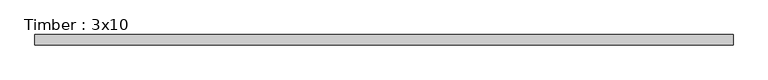
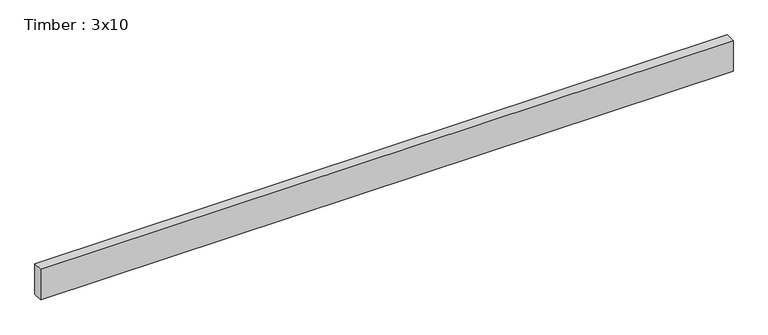
"""IFC4 building model written with IfcOpenShell, lengths in millimetres: beam geometry, Timber : 3x10."""

import ifcopenshell
import ifcopenshell.guid

model = None  # the IFC model being written
_history = None  # IfcOwnerHistory: only IFC2X3 demands one
_inside = {}  # id of a spatial element -> (the spatial element, [elements in it])
_under = {}  # id of a project, library or spatial element -> (it, [spatial elements below it])
_declared = {}  # id of a project -> (the project, [libraries it declares])
_typed = {}  # id of a type object -> (the type object, [elements of that type])
_made_of = {}  # id of a material, layer set ... -> (it, [elements and type objects made of it])


def new_model(schema):
    """Start an empty IFC model of exactly this schema.

    Asked for "IFC4X3", IfcOpenShell would pick the latest addendum, in which some entities
    have other attributes; the version numbers below select the first issue.
    IFC2X3 requires an IfcOwnerHistory on every rooted entity: one is made here for all.
    """
    global model, _history
    if schema == "IFC4X3":
        model = ifcopenshell.file(schema_version=(4, 3, 0, 0))
    else:
        model = ifcopenshell.file(schema=schema)
    _inside.clear()
    _under.clear()
    _declared.clear()
    _typed.clear()
    _made_of.clear()
    _history = None
    if model.schema == "IFC2X3":
        org = make("IfcOrganization", Name="unknown")
        user = make(
            "IfcPersonAndOrganization",
            ThePerson=make("IfcPerson", FamilyName="unknown"),
            TheOrganization=org,
        )
        app = make(
            "IfcApplication",
            ApplicationDeveloper=org,
            Version="unknown",
            ApplicationFullName="unknown",
            ApplicationIdentifier="unknown",
        )
        _history = make(
            "IfcOwnerHistory",
            OwningUser=user,
            OwningApplication=app,
            ChangeAction="ADDED",
            CreationDate=0,
        )
    return model


def make(cls, **values):
    """One entity of the class cls with the attributes given. An attribute that is None is left unset."""
    return model.create_entity(
        cls, **{name: value for name, value in values.items() if value is not None}
    )


def rooted(cls, **values):
    """An entity with a GlobalId (a new one), such as an element, a storey or a relation."""
    return make(cls, GlobalId=ifcopenshell.guid.new(), OwnerHistory=_history, **values)


def si_unit(unit_type, name, prefix=None):
    """IfcSIUnit, for example si_unit("LENGTHUNIT", "METRE", prefix="MILLI")."""
    return make("IfcSIUnit", UnitType=unit_type, Prefix=prefix, Name=name)


def assignment(units):
    """IfcUnitAssignment: the units of a project."""
    return None if units is None else make("IfcUnitAssignment", Units=units)


def point(xyz):
    """IfcCartesianPoint."""
    return None if xyz is None else make("IfcCartesianPoint", Coordinates=xyz)


def direction(xyz):
    """IfcDirection."""
    return None if xyz is None else make("IfcDirection", DirectionRatios=xyz)


def frame(location, z_axis=None, x_axis=None):
    """IfcAxis2Placement3D, a coordinate frame: its origin and axes. An axis left out is left unset."""
    return make(
        "IfcAxis2Placement3D",
        Location=point(location),
        Axis=direction(z_axis),
        RefDirection=direction(x_axis),
    )


def origin():
    """The frame at (0, 0, 0) with its axes left unset."""
    return frame((0.0, 0.0, 0.0))


def place(relative_to, where):
    """IfcLocalPlacement: puts the frame where relative to a parent placement (None: the world)."""
    return make(
        "IfcLocalPlacement", PlacementRelTo=relative_to, RelativePlacement=where
    )


def context(
    kind, dimensions, precision=None, world=None, true_north=None, identifier=None
):
    """IfcGeometricRepresentationContext, for example the 3D "Model" context."""
    return make(
        "IfcGeometricRepresentationContext",
        ContextIdentifier=identifier,
        ContextType=kind,
        CoordinateSpaceDimension=dimensions,
        Precision=precision,
        WorldCoordinateSystem=world,
        TrueNorth=true_north,
    )


def project(units=None, contexts=None):
    """IfcProject with its units and contexts."""
    return rooted(
        "IfcProject",
        Name="project",
        RepresentationContexts=contexts,
        UnitsInContext=assignment(units),
    )


def spatial(cls, under=None, at=None, **own):
    """A site, building, storey or space (cls), placed at a placement, below another one or the project."""
    s = rooted(cls, ObjectPlacement=at, **own)
    if under is not None:
        _under.setdefault(under.id(), (under, []))[1].append(s)
    return s


def polyline(points):
    """IfcPolyline through the points."""
    return make("IfcPolyline", Points=[point(p) for p in points])


def outline(outer, holes=None, kind="AREA"):
    """IfcArbitraryClosedProfileDef: a profile drawn as a closed curve; with holes, ...WithVoids."""
    if holes is None:
        return make("IfcArbitraryClosedProfileDef", ProfileType=kind, OuterCurve=outer)
    return make(
        "IfcArbitraryProfileDefWithVoids",
        ProfileType=kind,
        OuterCurve=outer,
        InnerCurves=holes,
    )


def extrude(swept, where, along, depth):
    """IfcExtrudedAreaSolid: the profile swept, set in the frame where, extruded along a direction by depth."""
    return make(
        "IfcExtrudedAreaSolid",
        SweptArea=swept,
        Position=where,
        ExtrudedDirection=direction(along),
        Depth=depth,
    )


def shape(context_of_items, identifier, shape_type, items):
    """IfcShapeRepresentation: the items that make up one representation, for example the "Body"."""
    return make(
        "IfcShapeRepresentation",
        ContextOfItems=context_of_items,
        RepresentationIdentifier=identifier,
        RepresentationType=shape_type,
        Items=items,
    )


def source(mapping_origin, context_of_items, identifier, shape_type, items):
    """IfcRepresentationMap: a shape defined once, which mapped items show again and again."""
    return make(
        "IfcRepresentationMap",
        MappingOrigin=mapping_origin,
        MappedRepresentation=shape(context_of_items, identifier, shape_type, items),
    )


def transform(
    local_origin,
    x_axis=None,
    y_axis=None,
    z_axis=None,
    scale=None,
    scale2=None,
    scale3=None,
    uniform=True,
):
    """IfcCartesianTransformationOperator3D, or its non-uniform kind. x_axis, y_axis, z_axis: its Axis1, 2, 3."""
    if uniform:
        return make(
            "IfcCartesianTransformationOperator3D",
            Axis1=direction(x_axis),
            Axis2=direction(y_axis),
            LocalOrigin=point(local_origin),
            Scale=scale,
            Axis3=direction(z_axis),
        )
    return make(
        "IfcCartesianTransformationOperator3DnonUniform",
        Axis1=direction(x_axis),
        Axis2=direction(y_axis),
        LocalOrigin=point(local_origin),
        Scale=scale,
        Axis3=direction(z_axis),
        Scale2=scale2,
        Scale3=scale3,
    )


def mapped(mapping_source, mapping_target):
    """IfcMappedItem: shows the shape of a source again, moved by a transform."""
    return make(
        "IfcMappedItem", MappingSource=mapping_source, MappingTarget=mapping_target
    )


def made_of(thing, what):
    """Note that an element or type object is made of a material, layer set ...; save() writes the relation."""
    if what is not None:
        _made_of.setdefault(what.id(), (what, []))[1].append(thing)
    return thing


def element(
    cls,
    number,
    at=None,
    inside=None,
    cuts=None,
    type_object=None,
    material=None,
    context=None,
    identifier="Body",
    shape_type=None,
    held_by="IfcProductDefinitionShape",
    body=None,
    shapes=None,
    **own,
):
    """One element of the class cls, such as IfcWall. Its Tag is "e" and its number.

    at: its placement. inside: the storey or other place that contains it. cuts: it is an
    opening in that element (IfcRelVoidsElement). A single representation is given by context,
    identifier, shape_type and body (its items); several are given by shapes. held_by: the class
    of the entity that holds the representations. save() writes the other relations.
    """
    e = rooted(cls, Tag="e%d" % number, ObjectPlacement=at, **own)
    if body is not None:
        shapes = [shape(context, identifier, shape_type, body)]
    if shapes is not None:
        e.Representation = make(held_by, Representations=shapes)
    if inside is not None:
        _inside.setdefault(inside.id(), (inside, []))[1].append(e)
    if cuts is not None:
        rooted(
            "IfcRelVoidsElement", RelatingBuildingElement=cuts, RelatedOpeningElement=e
        )
    if type_object is not None:
        _typed.setdefault(type_object.id(), (type_object, []))[1].append(e)
    return made_of(e, material)


def aggregate(whole, parts):
    """IfcRelAggregates: a whole, such as a stair, and the parts it consists of."""
    return rooted("IfcRelAggregates", RelatingObject=whole, RelatedObjects=parts)


def save(model, path):
    """Write the relations noted so far, then the file.

    IfcRelAggregates (storeys below a building ...), IfcRelContainedInSpatialStructure (elements
    in a storey), IfcRelDefinesByType, IfcRelAssociatesMaterial and IfcRelDeclares: one each for
    every whole, place, type object, material and project.
    """
    for whole, parts in _under.values():
        aggregate(whole, parts)
    for where, things in _inside.values():
        rooted(
            "IfcRelContainedInSpatialStructure",
            RelatedElements=things,
            RelatingStructure=where,
        )
    for kind, things in _typed.values():
        rooted("IfcRelDefinesByType", RelatedObjects=things, RelatingType=kind)
    for what, things in _made_of.values():
        rooted("IfcRelAssociatesMaterial", RelatedObjects=things, RelatingMaterial=what)
    for by, libraries in _declared.values():
        rooted("IfcRelDeclares", RelatingContext=by, RelatedDefinitions=libraries)
    model.write(path)


def timber_3x10_eec112f8(model_context):
    return source(origin(), model_context, "Body", "SweptSolid", [
        extrude(outline(polyline([(2565.4, 38.1), (2565.4, -38.1), (-2641.6, -38.1), (-2641.6, 38.1), (2565.4, 38.1)])), frame((0.0, 0.0, -120.65), z_axis=(0.0, 0.0, 1.0), x_axis=(1.0, 0.0, 0.0)), (0.0, 0.0, 1.0), 241.3),
    ])


if __name__ == "__main__":
    model = new_model("IFC4")
    model_context = context("Model", 3, world=origin())
    ifc_project = project(units=[si_unit("LENGTHUNIT", "METRE", prefix="MILLI")], contexts=[model_context])
    site = spatial("IfcSite", under=ifc_project)
    building = spatial("IfcBuilding", under=site)
    placement = place(None, origin())
    timber_3x10_shape = timber_3x10_eec112f8(model_context)
    element("IfcBeam", 1, ObjectType="Timber : 3x10", at=placement, inside=building, context=model_context, shape_type="MappedRepresentation", body=[
        mapped(timber_3x10_shape, transform((0.0, 0.0, 0.0), x_axis=(1.0, 0.0, 0.0), y_axis=(0.0, 1.0, 0.0), z_axis=(0.0, 0.0, 1.0))),
    ])
    save(model, "model.ifc")

# Revit data of these elements
# Type "Timber : 3x10"
#   Assembly Code = "B10"
#   A = 0.362847 SF
#   Length [instance default] = 5' - 0"
#   b = 0' - 3"
#   d = 0' - 9 1/2"
#   Structural Material [instance default] = Softwood, Lumber
# Element 1 (IfcBeam, "Timber : 3x10")
#   Materials on its faces: "Softwood, Lumber"
# Materials
#   "Softwood, Lumber": class "Wood", colour RGB 144 113 62, transparency 0, Description = "Pinus Echinata", Cost = 0
